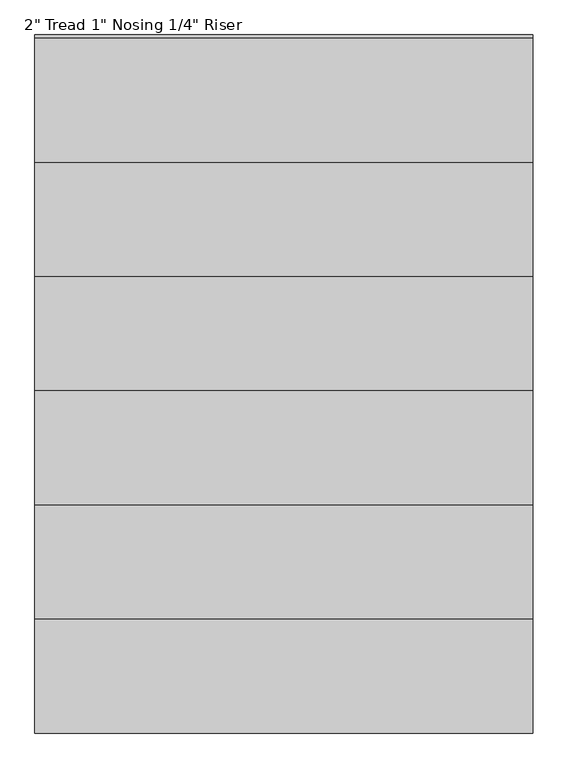
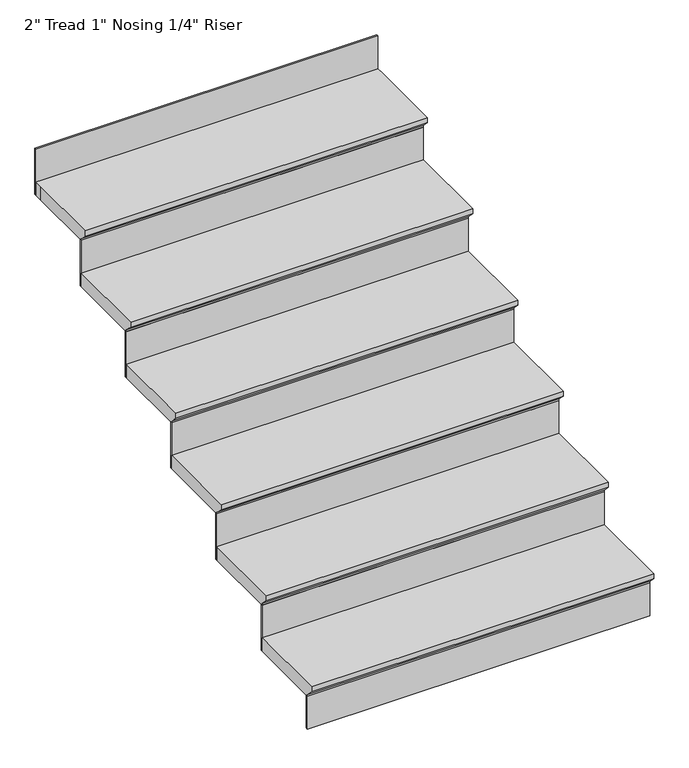
"""IFC4 building model written with IfcOpenShell, lengths in millimetres: stair flight geometry."""

from ifc_helpers import new_model, si_unit, origin, place, context, project, spatial, faceted_brep, source, transform, mapped, element, save


def stair_flight_3ac1b4c9(model_context):
    return source(origin(), model_context, "Body", "Brep", [
        faceted_brep([(-3020.5507921, -6344.8601743, 155.1214286), (-3020.5507921, -6344.8601743, 174.1714286), (-4239.7507921, -6344.8601743, 174.1714286), (-4239.7507921, -6344.8601743, 155.1214286), (-3020.5507921, -6319.4601743, 129.7214286), (-4239.7507921, -6319.4601743, 129.7214286), (-3020.5507921, -6040.0601743, 174.1714286), (-4239.7507921, -6040.0601743, 174.1714286), (-4239.7507921, -6319.4601743, 123.3714286), (-4239.7507921, -6040.0601743, 123.3714286), (-3020.5507921, -6040.0601743, 123.3714286), (-3020.5507921, -6319.4601743, 123.3714286)], [[[0, 1, 2, 3]], [[4, 0, 3, 5]], [[2, 1, 6, 7]], [[8, 9, 10, 11]], [[2, 7, 9, 8, 5, 3]], [[8, 11, 4, 5]], [[6, 1, 0, 4, 11, 10]], [[7, 6, 10, 9]]]),
        faceted_brep([(-3020.5507921, -6319.4601743, 123.3714286), (-3020.5507921, -6319.4601743, 0.0), (-3020.5507921, -6313.1101743, 0.0), (-3020.5507921, -6313.1101743, 123.3714286), (-4239.7507921, -6319.4601743, 123.3714286), (-4239.7507921, -6313.1101743, 123.3714286), (-4239.7507921, -6313.1101743, 0.0), (-4239.7507921, -6319.4601743, 0.0)], [[[0, 1, 2, 3]], [[4, 5, 6, 7]], [[1, 0, 4, 7]], [[2, 1, 7, 6]], [[3, 2, 6, 5]], [[0, 3, 5, 4]]]),
        faceted_brep([(-3020.5507921, -6040.0601743, 297.5428571), (-3020.5507921, -6040.0601743, 123.3714286), (-3020.5507921, -6033.7101743, 123.3714286), (-3020.5507921, -6033.7101743, 297.5428571), (-4239.7507921, -6040.0601743, 297.5428571), (-4239.7507921, -6033.7101743, 297.5428571), (-4239.7507921, -6033.7101743, 123.3714286), (-4239.7507921, -6040.0601743, 123.3714286)], [[[0, 1, 2, 3]], [[4, 5, 6, 7]], [[1, 0, 4, 7]], [[2, 1, 7, 6]], [[3, 2, 6, 5]], [[0, 3, 5, 4]]]),
        faceted_brep([(-4239.7507921, -6065.4601743, 348.3428571), (-3020.5507921, -6065.4601743, 348.3428571), (-3020.5507921, -5760.6601743, 348.3428571), (-4239.7507921, -5760.6601743, 348.3428571), (-4239.7507921, -6040.0601743, 297.5428571), (-4239.7507921, -5760.6601743, 297.5428571), (-3020.5507921, -5760.6601743, 297.5428571), (-3020.5507921, -6040.0601743, 297.5428571), (-4239.7507921, -6040.0601743, 303.8928571), (-4239.7507921, -6065.4601743, 329.2928571), (-3020.5507921, -6040.0601743, 303.8928571), (-3020.5507921, -6065.4601743, 329.2928571)], [[[0, 1, 2, 3]], [[4, 5, 6, 7]], [[0, 3, 5, 4, 8, 9]], [[4, 7, 10, 8]], [[2, 1, 11, 10, 7, 6]], [[3, 2, 6, 5]], [[11, 1, 0, 9]], [[10, 11, 9, 8]]]),
        faceted_brep([(-3020.5507921, -5760.6601743, 471.7142857), (-3020.5507921, -5760.6601743, 297.5428571), (-3020.5507921, -5754.3101743, 297.5428571), (-3020.5507921, -5754.3101743, 471.7142857), (-4239.7507921, -5760.6601743, 471.7142857), (-4239.7507921, -5754.3101743, 471.7142857), (-4239.7507921, -5754.3101743, 297.5428571), (-4239.7507921, -5760.6601743, 297.5428571)], [[[0, 1, 2, 3]], [[4, 5, 6, 7]], [[1, 0, 4, 7]], [[2, 1, 7, 6]], [[3, 2, 6, 5]], [[0, 3, 5, 4]]]),
        faceted_brep([(-4239.7507921, -5786.0601743, 522.5142857), (-3020.5507921, -5786.0601743, 522.5142857), (-3020.5507921, -5481.2601743, 522.5142857), (-4239.7507921, -5481.2601743, 522.5142857), (-4239.7507921, -5760.6601743, 471.7142857), (-4239.7507921, -5481.2601743, 471.7142857), (-3020.5507921, -5481.2601743, 471.7142857), (-3020.5507921, -5760.6601743, 471.7142857), (-4239.7507921, -5760.6601743, 478.0642857), (-4239.7507921, -5786.0601743, 503.4642857), (-3020.5507921, -5760.6601743, 478.0642857), (-3020.5507921, -5786.0601743, 503.4642857)], [[[0, 1, 2, 3]], [[4, 5, 6, 7]], [[0, 3, 5, 4, 8, 9]], [[4, 7, 10, 8]], [[2, 1, 11, 10, 7, 6]], [[3, 2, 6, 5]], [[11, 1, 0, 9]], [[10, 11, 9, 8]]]),
        faceted_brep([(-3020.5507921, -5481.2601743, 645.8857143), (-3020.5507921, -5481.2601743, 471.7142857), (-3020.5507921, -5474.9101743, 471.7142857), (-3020.5507921, -5474.9101743, 645.8857143), (-4239.7507921, -5481.2601743, 645.8857143), (-4239.7507921, -5474.9101743, 645.8857143), (-4239.7507921, -5474.9101743, 471.7142857), (-4239.7507921, -5481.2601743, 471.7142857)], [[[0, 1, 2, 3]], [[4, 5, 6, 7]], [[1, 0, 4, 7]], [[2, 1, 7, 6]], [[3, 2, 6, 5]], [[0, 3, 5, 4]]]),
        faceted_brep([(-4239.7507921, -5506.6601743, 696.6857143), (-3020.5507921, -5506.6601743, 696.6857143), (-3020.5507921, -5201.8601743, 696.6857143), (-4239.7507921, -5201.8601743, 696.6857143), (-4239.7507921, -5481.2601743, 645.8857143), (-4239.7507921, -5201.8601743, 645.8857143), (-3020.5507921, -5201.8601743, 645.8857143), (-3020.5507921, -5481.2601743, 645.8857143), (-4239.7507921, -5481.2601743, 652.2357143), (-4239.7507921, -5506.6601743, 677.6357143), (-3020.5507921, -5481.2601743, 652.2357143), (-3020.5507921, -5506.6601743, 677.6357143)], [[[0, 1, 2, 3]], [[4, 5, 6, 7]], [[0, 3, 5, 4, 8, 9]], [[4, 7, 10, 8]], [[2, 1, 11, 10, 7, 6]], [[3, 2, 6, 5]], [[11, 1, 0, 9]], [[10, 11, 9, 8]]]),
        faceted_brep([(-3020.5507921, -5201.8601743, 820.0571429), (-3020.5507921, -5201.8601743, 645.8857143), (-3020.5507921, -5195.5101743, 645.8857143), (-3020.5507921, -5195.5101743, 820.0571429), (-4239.7507921, -5201.8601743, 820.0571429), (-4239.7507921, -5195.5101743, 820.0571429), (-4239.7507921, -5195.5101743, 645.8857143), (-4239.7507921, -5201.8601743, 645.8857143)], [[[0, 1, 2, 3]], [[4, 5, 6, 7]], [[1, 0, 4, 7]], [[2, 1, 7, 6]], [[3, 2, 6, 5]], [[0, 3, 5, 4]]]),
        faceted_brep([(-4239.7507921, -5227.2601743, 870.8571429), (-3020.5507921, -5227.2601743, 870.8571429), (-3020.5507921, -4922.4601743, 870.8571429), (-4239.7507921, -4922.4601743, 870.8571429), (-4239.7507921, -5201.8601743, 820.0571429), (-4239.7507921, -4922.4601743, 820.0571429), (-3020.5507921, -4922.4601743, 820.0571429), (-3020.5507921, -5201.8601743, 820.0571429), (-4239.7507921, -5201.8601743, 826.4071429), (-4239.7507921, -5227.2601743, 851.8071429), (-3020.5507921, -5201.8601743, 826.4071429), (-3020.5507921, -5227.2601743, 851.8071429)], [[[0, 1, 2, 3]], [[4, 5, 6, 7]], [[0, 3, 5, 4, 8, 9]], [[4, 7, 10, 8]], [[2, 1, 11, 10, 7, 6]], [[3, 2, 6, 5]], [[11, 1, 0, 9]], [[10, 11, 9, 8]]]),
        faceted_brep([(-3020.5507921, -4922.4601743, 994.2285714), (-3020.5507921, -4922.4601743, 820.0571429), (-3020.5507921, -4916.1101743, 820.0571429), (-3020.5507921, -4916.1101743, 994.2285714), (-4239.7507921, -4922.4601743, 994.2285714), (-4239.7507921, -4916.1101743, 994.2285714), (-4239.7507921, -4916.1101743, 820.0571429), (-4239.7507921, -4922.4601743, 820.0571429)], [[[0, 1, 2, 3]], [[4, 5, 6, 7]], [[1, 0, 4, 7]], [[2, 1, 7, 6]], [[3, 2, 6, 5]], [[0, 3, 5, 4]]]),
        faceted_brep([(-3020.5507921, -4643.0601743, 1168.4), (-3020.5507921, -4643.0601743, 994.2285714), (-3020.5507921, -4636.7101743, 994.2285714), (-3020.5507921, -4636.7101743, 1168.4), (-4239.7507921, -4643.0601743, 1168.4), (-4239.7507921, -4636.7101743, 1168.4), (-4239.7507921, -4636.7101743, 994.2285714), (-4239.7507921, -4643.0601743, 994.2285714)], [[[0, 1, 2, 3]], [[4, 5, 6, 7]], [[1, 0, 4, 7]], [[2, 1, 7, 6]], [[3, 2, 6, 5]], [[0, 3, 5, 4]]]),
        faceted_brep([(-4239.7507921, -4643.0601743, 1045.0285714), (-4239.7507921, -4668.4601743, 1045.0285714), (-4239.7507921, -4947.8601743, 1045.0285714), (-3020.5507921, -4947.8601743, 1045.0285714), (-3020.5507921, -4668.4601743, 1045.0285714), (-3020.5507921, -4643.0601743, 1045.0285714), (-4239.7507921, -4668.4601743, 994.2285714), (-4239.7507921, -4643.0601743, 994.2285714), (-3020.5507921, -4643.0601743, 994.2285714), (-3020.5507921, -4668.4601743, 994.2285714), (-3020.5507921, -4922.4601743, 994.2285714), (-4239.7507921, -4922.4601743, 994.2285714), (-3020.5507921, -4922.4601743, 1000.5785714), (-4239.7507921, -4922.4601743, 1000.5785714), (-3020.5507921, -4947.8601743, 1025.9785714), (-4239.7507921, -4947.8601743, 1025.9785714)], [[[0, 1, 2, 3, 4, 5]], [[6, 7, 8, 9, 10, 11]], [[1, 0, 7, 6]], [[11, 10, 12, 13]], [[4, 3, 14, 12, 10, 9]], [[5, 4, 9, 8]], [[0, 5, 8, 7]], [[14, 3, 2, 15]], [[12, 14, 15, 13]], [[2, 1, 6, 11, 13, 15]]]),
    ])


if __name__ == "__main__":
    model = new_model("IFC4")
    model_context = context("Model", 3, world=origin())
    ifc_project = project(units=[si_unit("LENGTHUNIT", "METRE", prefix="MILLI")], contexts=[model_context])
    site = spatial("IfcSite", under=ifc_project)
    building = spatial("IfcBuilding", under=site)
    placement = place(None, origin())
    stair_flight_shape = stair_flight_3ac1b4c9(model_context)
    element("IfcStairFlight", 1, ObjectType="2\" Tread 1\" Nosing 1/4\" Riser", at=placement, inside=building, context=model_context, shape_type="MappedRepresentation", body=[
        mapped(stair_flight_shape, transform((0.0, 0.0, 0.0), x_axis=(1.0, 0.0, 0.0), y_axis=(0.0, 1.0, 0.0), z_axis=(0.0, 0.0, 1.0))),
    ])
    save(model, "model.ifc")
